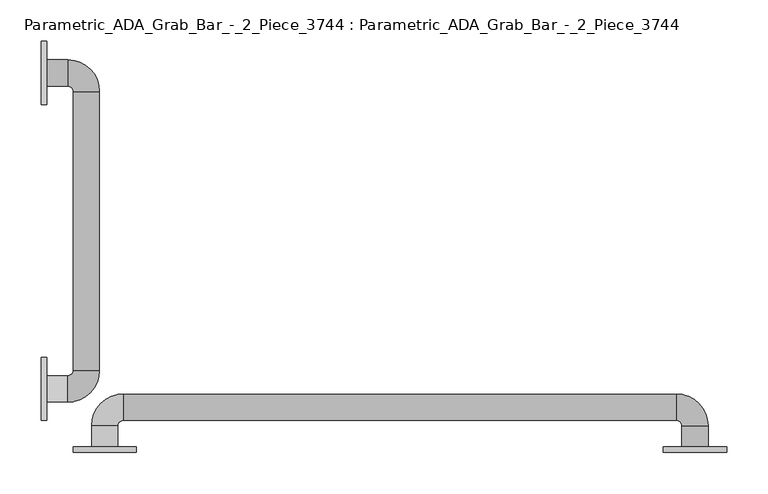
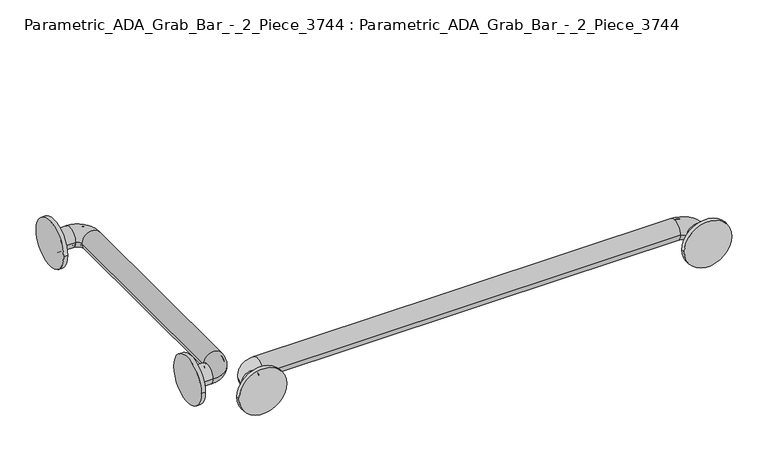
"""IFC4 building model written with IfcOpenShell, lengths in millimetres: proxy geometry, Parametric_ADA_Grab_Bar_-_2_Piece_3744 : Parametric_ADA_Grab_Bar_-_2_Piece_3744."""

from ifc_helpers import new_model, si_unit, point, frame, frame_2d, origin, place, context, project, spatial, polyline, circle_curve, ellipse_curve, trimmed, segment, composite_curve, outline, extrude, source, transform, mapped, element, save
from ifc_brep_helpers import plane_surface, cylinder_surface, revolved_surface, advanced_brep


def parametric_ada_grab_bar_2_piece_3744_parametric_ada_grab_bar_6f2753c4(model_context):
    return source(origin(), model_context, "Body", "SolidModel", [
        advanced_brep(
        [(6.35, 499.26875, 838.2), (6.35, 531.01875, 838.2), (6.35, 502.44375, 838.2), (6.35, 527.84375, 838.2), (31.75, 499.26875, 838.2), (31.75, 531.01875, 838.2), (31.75, 502.44375, 838.2), (31.75, 527.84375, 838.2), (69.85, 492.91875, 838.2), (38.1, 492.91875, 838.2), (66.675, 492.91875, 838.2), (41.275, 492.91875, 838.2), (38.1, 156.36875, 838.2), (69.85, 156.36875, 838.2), (41.275, 156.36875, 838.2), (66.675, 156.36875, 838.2), (31.75, 118.26875, 838.2), (31.75, 150.01875, 838.2), (31.75, 121.44375, 838.2), (31.75, 146.84375, 838.2), (6.35, 150.01875, 838.2), (6.35, 118.26875, 838.2), (6.35, 146.84375, 838.2), (6.35, 121.44375, 838.2)],
        [
            (0, 1, circle_curve(frame((6.35, 515.14375, 838.2), z_axis=(-1.0, 0.0, 0.0), x_axis=(0.0, 1.0, 0.0)), 15.875)),
            (1, 0, circle_curve(frame((6.35, 515.14375, 838.2), z_axis=(-1.0, 0.0, 0.0), x_axis=(0.0, 1.0, 0.0)), 15.875)),
            (2, 3, circle_curve(frame((6.35, 515.14375, 838.2), z_axis=(1.0, 0.0, 0.0), x_axis=(0.0, 1.0, 0.0)), 12.7)),
            (3, 2, circle_curve(frame((6.35, 515.14375, 838.2), z_axis=(1.0, 0.0, 0.0), x_axis=(0.0, 1.0, 0.0)), 12.7)),
            (0, 4),
            (4, 5, circle_curve(frame((31.75, 515.14375, 838.2), z_axis=(-1.0, 0.0, 0.0), x_axis=(0.0, 1.0, 0.0)), 15.875)),
            (5, 1),
            (5, 4, circle_curve(frame((31.75, 515.14375, 838.2), z_axis=(-1.0, 0.0, 0.0), x_axis=(0.0, 1.0, 0.0)), 15.875)),
            (2, 6),
            (6, 7, circle_curve(frame((31.75, 515.14375, 838.2), z_axis=(1.0, 0.0, 0.0), x_axis=(0.0, 1.0, 0.0)), 12.7)),
            (7, 3),
            (7, 6, circle_curve(frame((31.75, 515.14375, 838.2), z_axis=(1.0, 0.0, 0.0), x_axis=(0.0, 1.0, 0.0)), 12.7)),
            (8, 5, circle_curve(frame((31.75, 492.91875, 838.2), z_axis=(0.0, 0.0, 1.0), x_axis=(0.0, 1.0, 0.0)), 38.1)),
            (4, 9, circle_curve(frame((31.75, 492.91875, 838.2), z_axis=(0.0, 0.0, -1.0), x_axis=(0.0, 1.0, 0.0)), 6.35)),
            (9, 8, circle_curve(frame((53.975, 492.91875, 838.2), z_axis=(0.0, 1.0, 0.0), x_axis=(1.0, 0.0, 0.0)), 15.875)),
            (8, 9, circle_curve(frame((53.975, 492.91875, 838.2), z_axis=(0.0, 1.0, 0.0), x_axis=(1.0, 0.0, 0.0)), 15.875)),
            (10, 7, circle_curve(frame((31.75, 492.91875, 838.2), z_axis=(0.0, 0.0, 1.0), x_axis=(0.0, 1.0, 0.0)), 34.925)),
            (6, 11, circle_curve(frame((31.75, 492.91875, 838.2), z_axis=(0.0, 0.0, -1.0), x_axis=(0.0, 1.0, 0.0)), 9.525)),
            (11, 10, circle_curve(frame((53.975, 492.91875, 838.2), z_axis=(0.0, -1.0, 0.0), x_axis=(1.0, 0.0, 0.0)), 12.7)),
            (10, 11, circle_curve(frame((53.975, 492.91875, 838.2), z_axis=(0.0, -1.0, 0.0), x_axis=(1.0, 0.0, 0.0)), 12.7)),
            (9, 12),
            (12, 13, circle_curve(frame((53.975, 156.36875, 838.2), z_axis=(0.0, 1.0, 0.0), x_axis=(1.0, 0.0, 0.0)), 15.875)),
            (13, 8),
            (13, 12, circle_curve(frame((53.975, 156.36875, 838.2), z_axis=(0.0, 1.0, 0.0), x_axis=(1.0, 0.0, 0.0)), 15.875)),
            (11, 14),
            (14, 15, circle_curve(frame((53.975, 156.36875, 838.2), z_axis=(0.0, -1.0, 0.0), x_axis=(1.0, 0.0, 0.0)), 12.7)),
            (15, 10),
            (15, 14, circle_curve(frame((53.975, 156.36875, 838.2), z_axis=(0.0, -1.0, 0.0), x_axis=(1.0, 0.0, 0.0)), 12.7)),
            (16, 13, circle_curve(frame((31.75, 156.36875, 838.2), z_axis=(0.0, 0.0, 1.0), x_axis=(1.0, 0.0, 0.0)), 38.1)),
            (12, 17, circle_curve(frame((31.75, 156.36875, 838.2), z_axis=(0.0, 0.0, -1.0), x_axis=(1.0, 0.0, 0.0)), 6.35)),
            (17, 16, circle_curve(frame((31.75, 134.14375, 838.2), z_axis=(1.0, -1.0754999491619899e-12, 0.0), x_axis=(-1.0754999491619899e-12, -1.0, 0.0)), 15.875)),
            (16, 17, circle_curve(frame((31.75, 134.14375, 838.2), z_axis=(1.0, 0.0, 0.0), x_axis=(0.0, -1.0, 0.0)), 15.875)),
            (18, 15, circle_curve(frame((31.75, 156.36875, 838.2), z_axis=(0.0, 0.0, 1.0), x_axis=(1.0, 0.0, 0.0)), 34.925)),
            (14, 19, circle_curve(frame((31.75, 156.36875, 838.2), z_axis=(0.0, 0.0, -1.0), x_axis=(1.0, 0.0, 0.0)), 9.525)),
            (19, 18, circle_curve(frame((31.75, 134.14375, 838.2), z_axis=(-1.0, 0.0, 0.0), x_axis=(0.0, -1.0, 0.0)), 12.7)),
            (18, 19, circle_curve(frame((31.75, 134.14375, 838.2), z_axis=(-1.0, 0.0, 0.0), x_axis=(0.0, -1.0, 0.0)), 12.7)),
            (20, 21, circle_curve(frame((6.35, 134.14375, 838.2), z_axis=(-1.0, 0.0, 0.0), x_axis=(0.0, -1.0, 0.0)), 15.875)),
            (21, 20, circle_curve(frame((6.35, 134.14375, 838.2), z_axis=(-1.0, 0.0, 0.0), x_axis=(0.0, -1.0, 0.0)), 15.875)),
            (22, 23, circle_curve(frame((6.35, 134.14375, 838.2), z_axis=(1.0, 0.0, 0.0), x_axis=(0.0, -1.0, 0.0)), 12.7)),
            (23, 22, circle_curve(frame((6.35, 134.14375, 838.2), z_axis=(1.0, 0.0, 0.0), x_axis=(0.0, -1.0, 0.0)), 12.7)),
            (17, 20),
            (21, 16),
            (19, 22),
            (23, 18),
        ],
        [
            plane_surface(frame((6.35, 515.14375, 838.2), z_axis=(-1.0, 0.0, 0.0), x_axis=(0.0, 0.0, 1.0))),
            cylinder_surface(frame((6.35, 515.14375, 838.2), z_axis=(-1.0, 0.0, 0.0), x_axis=(0.0, 1.0, 0.0)), 15.875),
            revolved_surface(polyline([(31.75, 527.84375, 838.2), (6.35, 527.84375, 838.2)]), (6.35, 515.14375, 838.2), (1.0, 0.0, 0.0)),
            revolved_surface(trimmed(ellipse_curve(frame((31.75, 515.14375, 838.2), z_axis=(-1.0, 0.0, 0.0), x_axis=(0.0, 1.0, 0.0)), 15.875, 15.875), [point((31.75, 499.26875, 838.2))], [point((31.75, 531.01875, 838.2))], True, "CARTESIAN"), (31.75, 492.91875, 838.2), (0.0, 0.0, -1.0)),
            revolved_surface(trimmed(ellipse_curve(frame((31.75, 515.14375, 838.2), z_axis=(-1.0, 0.0, 0.0), x_axis=(0.0, 1.0, 0.0)), 15.875, 15.875), [point((31.75, 531.01875, 838.2))], [point((31.75, 499.26875, 838.2))], True, "CARTESIAN"), (31.75, 492.91875, 838.2), (0.0, 0.0, -1.0)),
            revolved_surface(trimmed(ellipse_curve(frame((31.75, 515.14375, 838.2), z_axis=(1.0, 0.0, 0.0), x_axis=(0.0, 1.0, 0.0)), 12.7, 12.7), [point((31.75, 502.44375, 838.2))], [point((31.75, 527.84375, 838.2))], True, "CARTESIAN"), (31.75, 492.91875, 838.2), (0.0, 0.0, -1.0)),
            revolved_surface(trimmed(ellipse_curve(frame((31.75, 515.14375, 838.2), z_axis=(1.0, 0.0, 0.0), x_axis=(0.0, 1.0, 0.0)), 12.7, 12.7), [point((31.75, 527.84375, 838.2))], [point((31.75, 502.44375, 838.2))], True, "CARTESIAN"), (31.75, 492.91875, 838.2), (0.0, 0.0, -1.0)),
            cylinder_surface(frame((53.975, 492.91875, 838.2), z_axis=(0.0, 1.0, 0.0), x_axis=(1.0, 0.0, 0.0)), 15.875),
            revolved_surface(polyline([(66.675, 156.36875000000003, 838.2), (66.675, 492.91875, 838.2)]), (53.975, 492.91875, 838.2), (0.0, -1.0, 0.0)),
            revolved_surface(trimmed(ellipse_curve(frame((53.975, 156.36875, 838.2), z_axis=(0.0, 1.0, 0.0), x_axis=(1.0, 0.0, 0.0)), 15.875, 15.875), [point((38.1, 156.36875, 838.2))], [point((69.85, 156.36875, 838.2))], True, "CARTESIAN"), (31.75, 156.36875, 838.2), (0.0, 0.0, -1.0)),
            revolved_surface(trimmed(ellipse_curve(frame((53.975, 156.36875, 838.2), z_axis=(0.0, 1.0, 0.0), x_axis=(1.0, 0.0, 0.0)), 15.875, 15.875), [point((69.85, 156.36875, 838.2))], [point((38.1, 156.36875, 838.2))], True, "CARTESIAN"), (31.75, 156.36875, 838.2), (0.0, 0.0, -1.0)),
            revolved_surface(trimmed(ellipse_curve(frame((53.975, 156.36875, 838.2), z_axis=(0.0, -1.0, 0.0), x_axis=(1.0, 0.0, 0.0)), 12.7, 12.7), [point((41.275, 156.36875, 838.2))], [point((66.675, 156.36875, 838.2))], True, "CARTESIAN"), (31.75, 156.36875, 838.2), (0.0, 0.0, -1.0)),
            revolved_surface(trimmed(ellipse_curve(frame((53.975, 156.36875, 838.2), z_axis=(0.0, -1.0, 0.0), x_axis=(1.0, 0.0, 0.0)), 12.7, 12.7), [point((66.675, 156.36875, 838.2))], [point((41.275, 156.36875, 838.2))], True, "CARTESIAN"), (31.75, 156.36875, 838.2), (0.0, 0.0, -1.0)),
            plane_surface(frame((6.35, 134.14375, 838.2), z_axis=(-1.0, 0.0, 0.0), x_axis=(0.0, 0.0, 1.0))),
            cylinder_surface(frame((31.75, 134.14375, 838.2), z_axis=(1.0, 0.0, 0.0), x_axis=(0.0, -1.0, 0.0)), 15.875),
            revolved_surface(polyline([(6.350000000000001, 121.44375000000001, 838.2), (31.75, 121.44375000000001, 838.2)]), (31.75, 134.14375, 838.2), (-1.0, 0.0, 0.0)),
        ],
        [
            (0, [[1, 2], [3, 4]]),
            (1, [[-1, 5, 6, 7]]),
            (1, [[-2, -7, 8, -5]]),
            (2, [[-3, 9, 10, 11]]),
            (2, [[-4, -11, 12, -9]]),
            (3, [[13, -6, 14, 15]]),
            (4, [[-14, -8, -13, 16]]),
            (5, [[17, -10, 18, 19]]),
            (6, [[-18, -12, -17, 20]]),
            (7, [[-15, 21, 22, 23]]),
            (7, [[-16, -23, 24, -21]]),
            (8, [[-19, 25, 26, 27]]),
            (8, [[-20, -27, 28, -25]]),
            (9, [[29, -22, 30, 31]]),
            (10, [[-30, -24, -29, 32]]),
            (11, [[33, -26, 34, 35]]),
            (12, [[-34, -28, -33, 36]]),
            (13, [[37, 38], [39, 40]]),
            (14, [[-31, 41, -38, 42]]),
            (14, [[-32, -42, -37, -41]]),
            (15, [[-35, 43, -40, 44]]),
            (15, [[-36, -44, -39, -43]]),
        ],
    ),
        advanced_brep(
        [(92.075, 64.29375, 838.2), (60.325, 64.29375, 838.2), (88.9, 64.29375, 838.2), (63.5, 64.29375, 838.2), (92.075, 89.69375, 838.2), (60.325, 89.69375, 838.2), (88.9, 89.69375, 838.2), (63.5, 89.69375, 838.2), (98.425, 127.79375, 838.2), (98.425, 96.04375, 838.2), (98.425, 124.61875, 838.2), (98.425, 99.21875, 838.2), (765.175, 96.04375, 838.2), (765.175, 127.79375, 838.2), (765.175, 99.21875, 838.2), (765.175, 124.61875, 838.2), (803.275, 89.69375, 838.2), (771.525, 89.69375, 838.2), (800.1, 89.69375, 838.2), (774.7, 89.69375, 838.2), (771.525, 64.29375, 838.2), (803.275, 64.29375, 838.2), (774.7, 64.29375, 838.2), (800.1, 64.29375, 838.2)],
        [
            (0, 1, circle_curve(frame((76.2, 64.29375, 838.2), z_axis=(0.0, -1.0, 0.0), x_axis=(-1.0, 0.0, 0.0)), 15.875)),
            (1, 0, circle_curve(frame((76.2, 64.29375, 838.2), z_axis=(0.0, -1.0, 0.0), x_axis=(-1.0, 0.0, 0.0)), 15.875)),
            (2, 3, circle_curve(frame((76.2, 64.29375, 838.2), z_axis=(0.0, 1.0, 0.0), x_axis=(-1.0, 0.0, 0.0)), 12.7)),
            (3, 2, circle_curve(frame((76.2, 64.29375, 838.2), z_axis=(0.0, 1.0, 0.0), x_axis=(-1.0, 0.0, 0.0)), 12.7)),
            (0, 4),
            (4, 5, circle_curve(frame((76.2, 89.69375, 838.2), z_axis=(0.0, -1.0, 0.0), x_axis=(-1.0, 0.0, 0.0)), 15.875)),
            (5, 1),
            (5, 4, circle_curve(frame((76.2, 89.69375, 838.2), z_axis=(0.0, -1.0, 0.0), x_axis=(-1.0, 0.0, 0.0)), 15.875)),
            (2, 6),
            (6, 7, circle_curve(frame((76.2, 89.69375, 838.2), z_axis=(0.0, 1.0, 0.0), x_axis=(-1.0, 0.0, 0.0)), 12.7)),
            (7, 3),
            (7, 6, circle_curve(frame((76.2, 89.69375, 838.2), z_axis=(0.0, 1.0, 0.0), x_axis=(-1.0, 0.0, 0.0)), 12.7)),
            (8, 5, circle_curve(frame((98.425, 89.69375, 838.2), z_axis=(0.0, 0.0, 1.0), x_axis=(-1.0, 0.0, 0.0)), 38.1)),
            (4, 9, circle_curve(frame((98.425, 89.69375, 838.2), z_axis=(0.0, 0.0, -1.0), x_axis=(-1.0, 0.0, 0.0)), 6.35)),
            (9, 8, circle_curve(frame((98.425, 111.91875, 838.2), z_axis=(-1.0, 0.0, 0.0), x_axis=(0.0, 1.0, 0.0)), 15.875)),
            (8, 9, circle_curve(frame((98.425, 111.91875, 838.2), z_axis=(-1.0, 0.0, 0.0), x_axis=(0.0, 1.0, 0.0)), 15.875)),
            (10, 7, circle_curve(frame((98.425, 89.69375, 838.2), z_axis=(0.0, 0.0, 1.0), x_axis=(-1.0, 0.0, 0.0)), 34.925)),
            (6, 11, circle_curve(frame((98.425, 89.69375, 838.2), z_axis=(0.0, 0.0, -1.0), x_axis=(-1.0, 0.0, 0.0)), 9.525)),
            (11, 10, circle_curve(frame((98.425, 111.91875, 838.2), z_axis=(1.0, 0.0, 0.0), x_axis=(0.0, 1.0, 0.0)), 12.7)),
            (10, 11, circle_curve(frame((98.425, 111.91875, 838.2), z_axis=(1.0, 0.0, 0.0), x_axis=(0.0, 1.0, 0.0)), 12.7)),
            (9, 12),
            (12, 13, circle_curve(frame((765.175, 111.91875, 838.2), z_axis=(-1.0, 0.0, 0.0), x_axis=(0.0, 1.0, 0.0)), 15.875)),
            (13, 8),
            (13, 12, circle_curve(frame((765.175, 111.91875, 838.2), z_axis=(-1.0, 0.0, 0.0), x_axis=(0.0, 1.0, 0.0)), 15.875)),
            (11, 14),
            (14, 15, circle_curve(frame((765.175, 111.91875, 838.2), z_axis=(1.0, 0.0, 0.0), x_axis=(0.0, 1.0, 0.0)), 12.7)),
            (15, 10),
            (15, 14, circle_curve(frame((765.175, 111.91875, 838.2), z_axis=(1.0, 0.0, 0.0), x_axis=(0.0, 1.0, 0.0)), 12.7)),
            (16, 13, circle_curve(frame((765.175, 89.69375, 838.2), z_axis=(0.0, 0.0, 1.0), x_axis=(0.0, 1.0, 0.0)), 38.1)),
            (12, 17, circle_curve(frame((765.175, 89.69375, 838.2), z_axis=(0.0, 0.0, -1.0), x_axis=(0.0, 1.0, 0.0)), 6.35)),
            (17, 16, circle_curve(frame((787.4, 89.69375, 838.2), z_axis=(1.0770542613964651e-12, 1.0, 0.0), x_axis=(1.0, -1.0770542613964651e-12, 0.0)), 15.875)),
            (16, 17, circle_curve(frame((787.4, 89.69375, 838.2), z_axis=(0.0, 1.0, 0.0), x_axis=(1.0, 0.0, 0.0)), 15.875)),
            (18, 15, circle_curve(frame((765.175, 89.69375, 838.2), z_axis=(0.0, 0.0, 1.0), x_axis=(0.0, 1.0, 0.0)), 34.925)),
            (14, 19, circle_curve(frame((765.175, 89.69375, 838.2), z_axis=(0.0, 0.0, -1.0), x_axis=(0.0, 1.0, 0.0)), 9.525)),
            (19, 18, circle_curve(frame((787.4, 89.69375, 838.2), z_axis=(0.0, -1.0, 0.0), x_axis=(1.0, 0.0, 0.0)), 12.7)),
            (18, 19, circle_curve(frame((787.4, 89.69375, 838.2), z_axis=(0.0, -1.0, 0.0), x_axis=(1.0, 0.0, 0.0)), 12.7)),
            (20, 21, circle_curve(frame((787.4, 64.29375, 838.2), z_axis=(0.0, -1.0, 0.0), x_axis=(1.0, 0.0, 0.0)), 15.875)),
            (21, 20, circle_curve(frame((787.4, 64.29375, 838.2), z_axis=(0.0, -1.0, 0.0), x_axis=(1.0, 0.0, 0.0)), 15.875)),
            (22, 23, circle_curve(frame((787.4, 64.29375, 838.2), z_axis=(0.0, 1.0, 0.0), x_axis=(1.0, 0.0, 0.0)), 12.7)),
            (23, 22, circle_curve(frame((787.4, 64.29375, 838.2), z_axis=(0.0, 1.0, 0.0), x_axis=(1.0, 0.0, 0.0)), 12.7)),
            (17, 20),
            (21, 16),
            (19, 22),
            (23, 18),
        ],
        [
            plane_surface(frame((76.2, 64.29375, 838.2), z_axis=(0.0, -1.0, 0.0), x_axis=(0.0, 0.0, 1.0))),
            cylinder_surface(frame((76.2, 64.29375, 838.2), z_axis=(0.0, -1.0, 0.0), x_axis=(-1.0, 0.0, 0.0)), 15.875),
            revolved_surface(polyline([(63.5, 89.69375, 838.2), (63.5, 64.29375, 838.2)]), (76.2, 64.29375, 838.2), (0.0, 1.0, 0.0)),
            revolved_surface(trimmed(ellipse_curve(frame((76.2, 89.69375, 838.2), z_axis=(0.0, -1.0, 0.0), x_axis=(-1.0, 0.0, 0.0)), 15.875, 15.875), [point((92.075, 89.69375, 838.2))], [point((60.325, 89.69375, 838.2))], True, "CARTESIAN"), (98.425, 89.69375, 838.2), (0.0, 0.0, -1.0)),
            revolved_surface(trimmed(ellipse_curve(frame((76.2, 89.69375, 838.2), z_axis=(0.0, -1.0, 0.0), x_axis=(-1.0, 0.0, 0.0)), 15.875, 15.875), [point((60.325, 89.69375, 838.2))], [point((92.075, 89.69375, 838.2))], True, "CARTESIAN"), (98.425, 89.69375, 838.2), (0.0, 0.0, -1.0)),
            revolved_surface(trimmed(ellipse_curve(frame((76.2, 89.69375, 838.2), z_axis=(0.0, 1.0, 0.0), x_axis=(-1.0, 0.0, 0.0)), 12.7, 12.7), [point((88.9, 89.69375, 838.2))], [point((63.5, 89.69375, 838.2))], True, "CARTESIAN"), (98.425, 89.69375, 838.2), (0.0, 0.0, -1.0)),
            revolved_surface(trimmed(ellipse_curve(frame((76.2, 89.69375, 838.2), z_axis=(0.0, 1.0, 0.0), x_axis=(-1.0, 0.0, 0.0)), 12.7, 12.7), [point((63.5, 89.69375, 838.2))], [point((88.9, 89.69375, 838.2))], True, "CARTESIAN"), (98.425, 89.69375, 838.2), (0.0, 0.0, -1.0)),
            cylinder_surface(frame((98.425, 111.91875, 838.2), z_axis=(-1.0, 0.0, 0.0), x_axis=(0.0, 1.0, 0.0)), 15.875),
            revolved_surface(polyline([(765.175, 124.61875, 838.2), (98.425, 124.61875, 838.2)]), (98.425, 111.91875, 838.2), (1.0, 0.0, 0.0)),
            revolved_surface(trimmed(ellipse_curve(frame((765.175, 111.91875, 838.2), z_axis=(-1.0, 0.0, 0.0), x_axis=(0.0, 1.0, 0.0)), 15.875, 15.875), [point((765.175, 96.04375, 838.2))], [point((765.175, 127.79375, 838.2))], True, "CARTESIAN"), (765.175, 89.69375, 838.2), (0.0, 0.0, -1.0)),
            revolved_surface(trimmed(ellipse_curve(frame((765.175, 111.91875, 838.2), z_axis=(-1.0, 0.0, 0.0), x_axis=(0.0, 1.0, 0.0)), 15.875, 15.875), [point((765.175, 127.79375, 838.2))], [point((765.175, 96.04375, 838.2))], True, "CARTESIAN"), (765.175, 89.69375, 838.2), (0.0, 0.0, -1.0)),
            revolved_surface(trimmed(ellipse_curve(frame((765.175, 111.91875, 838.2), z_axis=(1.0, 0.0, 0.0), x_axis=(0.0, 1.0, 0.0)), 12.7, 12.7), [point((765.175, 99.21875, 838.2))], [point((765.175, 124.61875, 838.2))], True, "CARTESIAN"), (765.175, 89.69375, 838.2), (0.0, 0.0, -1.0)),
            revolved_surface(trimmed(ellipse_curve(frame((765.175, 111.91875, 838.2), z_axis=(1.0, 0.0, 0.0), x_axis=(0.0, 1.0, 0.0)), 12.7, 12.7), [point((765.175, 124.61875, 838.2))], [point((765.175, 99.21875, 838.2))], True, "CARTESIAN"), (765.175, 89.69375, 838.2), (0.0, 0.0, -1.0)),
            plane_surface(frame((787.4, 64.29375, 838.2), z_axis=(0.0, -1.0, 0.0), x_axis=(0.0, 0.0, 1.0))),
            cylinder_surface(frame((787.4, 89.69375, 838.2), z_axis=(0.0, 1.0, 0.0), x_axis=(1.0, 0.0, 0.0)), 15.875),
            revolved_surface(polyline([(800.1, 64.29375, 838.2), (800.1, 89.69375, 838.2)]), (787.4, 89.69375, 838.2), (0.0, -1.0, 0.0)),
        ],
        [
            (0, [[1, 2], [3, 4]]),
            (1, [[-1, 5, 6, 7]]),
            (1, [[-2, -7, 8, -5]]),
            (2, [[-3, 9, 10, 11]]),
            (2, [[-4, -11, 12, -9]]),
            (3, [[13, -6, 14, 15]]),
            (4, [[-14, -8, -13, 16]]),
            (5, [[17, -10, 18, 19]]),
            (6, [[-18, -12, -17, 20]]),
            (7, [[-15, 21, 22, 23]]),
            (7, [[-16, -23, 24, -21]]),
            (8, [[-19, 25, 26, 27]]),
            (8, [[-20, -27, 28, -25]]),
            (9, [[29, -22, 30, 31]]),
            (10, [[-30, -24, -29, 32]]),
            (11, [[33, -26, 34, 35]]),
            (12, [[-34, -28, -33, 36]]),
            (13, [[37, 38], [39, 40]]),
            (14, [[-31, 41, -38, 42]]),
            (14, [[-32, -42, -37, -41]]),
            (15, [[-35, 43, -40, 44]]),
            (15, [[-36, -44, -39, -43]]),
        ],
    ),
        extrude(outline(composite_curve([segment(trimmed(circle_curve(frame_2d((134.14375, 838.2)), 38.1), [point((96.04375, 838.2))], [point((172.24375, 838.2))], False, "CARTESIAN"), True, "CONTINUOUS"), segment(trimmed(circle_curve(frame_2d((134.14375, 838.2)), 38.1), [point((172.24375, 838.2))], [point((96.04375, 838.2))], False, "CARTESIAN"), True, "CONTINUOUS")], self_intersect=False)), frame((0.0, 0.0, 0.0), z_axis=(1.0, 0.0, 0.0), x_axis=(0.0, 1.0, 0.0)), (0.0, 0.0, 1.0), 6.35),
        extrude(outline(composite_curve([segment(trimmed(circle_curve(frame_2d((515.14375, 838.2)), 38.1), [point((477.04375, 838.2))], [point((553.24375, 838.2))], False, "CARTESIAN"), True, "CONTINUOUS"), segment(trimmed(circle_curve(frame_2d((515.14375, 838.2)), 38.1), [point((553.24375, 838.2))], [point((477.04375, 838.2))], False, "CARTESIAN"), True, "CONTINUOUS")], self_intersect=False)), frame((0.0, 0.0, 0.0), z_axis=(1.0, 0.0, 0.0), x_axis=(0.0, 1.0, 0.0)), (0.0, 0.0, 1.0), 6.35),
        extrude(outline(composite_curve([segment(trimmed(circle_curve(frame_2d((838.2, 787.4)), 38.1), [point((838.2, 749.3))], [point((838.2, 825.5))], False, "CARTESIAN"), True, "CONTINUOUS"), segment(trimmed(circle_curve(frame_2d((838.2, 787.4)), 38.1), [point((838.2, 825.5))], [point((838.2, 749.3))], False, "CARTESIAN"), True, "CONTINUOUS")], self_intersect=False)), frame((0.0, 57.94375, 0.0), z_axis=(0.0, 1.0, 0.0), x_axis=(0.0, 0.0, 1.0)), (0.0, 0.0, 1.0), 6.35),
        extrude(outline(composite_curve([segment(trimmed(circle_curve(frame_2d((838.2, 76.2)), 38.1), [point((838.2, 38.1))], [point((838.2, 114.3))], False, "CARTESIAN"), True, "CONTINUOUS"), segment(trimmed(circle_curve(frame_2d((838.2, 76.2)), 38.1), [point((838.2, 114.3))], [point((838.2, 38.1))], False, "CARTESIAN"), True, "CONTINUOUS")], self_intersect=False)), frame((0.0, 57.94375, 0.0), z_axis=(0.0, 1.0, 0.0), x_axis=(0.0, 0.0, 1.0)), (0.0, 0.0, 1.0), 6.35),
    ])


if __name__ == "__main__":
    model = new_model("IFC4")
    model_context = context("Model", 3, world=origin())
    ifc_project = project(units=[si_unit("LENGTHUNIT", "METRE", prefix="MILLI")], contexts=[model_context])
    site = spatial("IfcSite", under=ifc_project)
    building = spatial("IfcBuilding", under=site)
    placement = place(None, origin())
    parametric_ada_grab_bar_2_piece_3744_parametric_ada_grab_bar_shape = parametric_ada_grab_bar_2_piece_3744_parametric_ada_grab_bar_6f2753c4(model_context)
    element("IfcBuildingElementProxy", 1, Name="Parametric_ADA_Grab_Bar_-_2_Piece_3744 : Parametric_ADA_Grab_Bar_-_2_Piece_3744", ObjectType="Parametric_ADA_Grab_Bar_-_2_Piece_3744 : Parametric_ADA_Grab_Bar_-_2_Piece_3744", at=placement, inside=building, context=model_context, shape_type="MappedRepresentation", body=[
        mapped(parametric_ada_grab_bar_2_piece_3744_parametric_ada_grab_bar_shape, transform((0.0, 0.0, 0.0), x_axis=(1.0, 0.0, 0.0), y_axis=(0.0, 1.0, 0.0), z_axis=(0.0, 0.0, 1.0))),
    ])
    save(model, "model.ifc")

# Revit data of these elements
# Project information
#   Project Issue Date = "07/20/2015"
#   Project Status = "Project Status"
#   Client Name = "Xcel"
#   Project Address = "Enter address here"
#   Project Name = "Xcel Sports Complex - Jefferson, WI"
#   Project Number = "Project Number"
# Type "Parametric_ADA_Grab_Bar_-_2_Piece_3744 : Parametric_ADA_Grab_Bar_-_2_Piece_3744"
#   Keynote = "M10281313.01"
#   Grab bar length (42" min) = 1' - 3"
#   Grab bar height = 2' - 9"
#   Grab bar Length (36" min) = 2' - 4"
#   Face of Wall to Grab bar (6" max) = 0' - 3"
#   Face of Wall to Grab bar (12" max) = 0' - 3"
# Element 1 (IfcBuildingElementProxy, "Parametric_ADA_Grab_Bar_-_2_Piece_3744 : Parametric_ADA_Grab_Bar_-_2_Piece_3744")
#   Materials on its faces: "Stainless Steel"
# Materials
#   "Stainless Steel": class "Metal", colour RGB 0 0 0, transparency 0, Description = "Stainless Steel 18/8", Cost = 0
